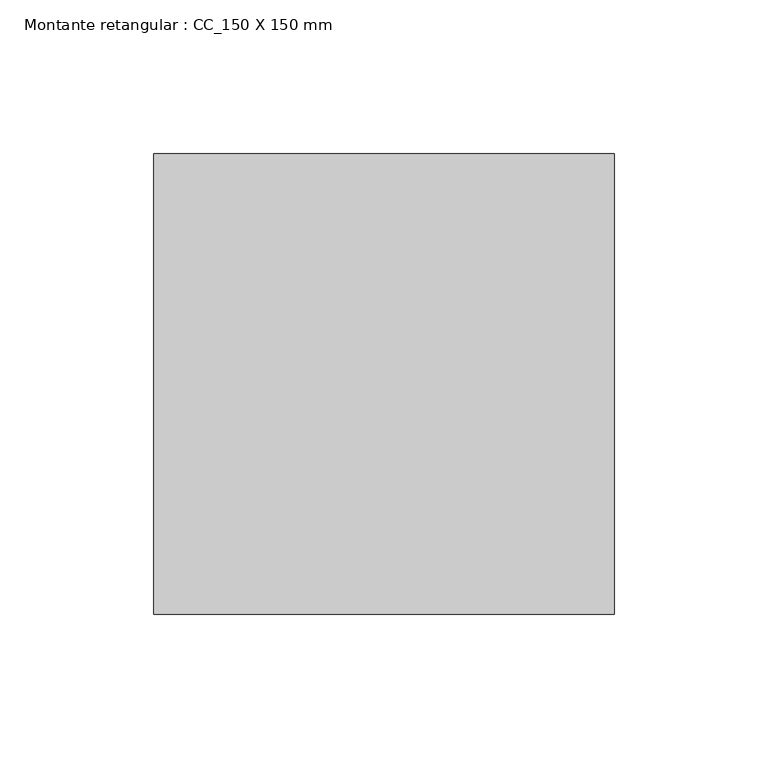
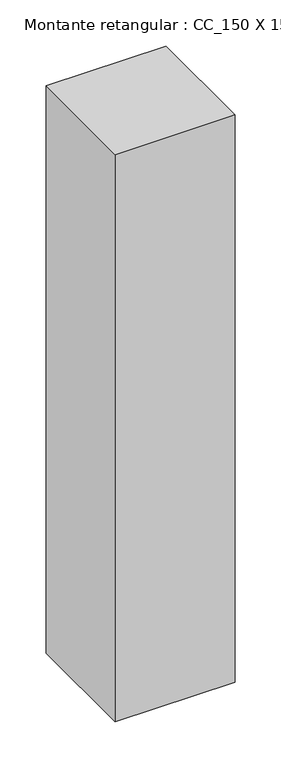
"""IFC4 building model written with IfcOpenShell, lengths in millimetres: member geometry, Montante retangular : CC_150 X 150 mm."""

import ifcopenshell
import ifcopenshell.guid

model = None  # the IFC model being written
_history = None  # IfcOwnerHistory: only IFC2X3 demands one
_inside = {}  # id of a spatial element -> (the spatial element, [elements in it])
_under = {}  # id of a project, library or spatial element -> (it, [spatial elements below it])
_declared = {}  # id of a project -> (the project, [libraries it declares])
_typed = {}  # id of a type object -> (the type object, [elements of that type])
_made_of = {}  # id of a material, layer set ... -> (it, [elements and type objects made of it])


def new_model(schema):
    """Start an empty IFC model of exactly this schema.

    Asked for "IFC4X3", IfcOpenShell would pick the latest addendum, in which some entities
    have other attributes; the version numbers below select the first issue.
    IFC2X3 requires an IfcOwnerHistory on every rooted entity: one is made here for all.
    """
    global model, _history
    if schema == "IFC4X3":
        model = ifcopenshell.file(schema_version=(4, 3, 0, 0))
    else:
        model = ifcopenshell.file(schema=schema)
    _inside.clear()
    _under.clear()
    _declared.clear()
    _typed.clear()
    _made_of.clear()
    _history = None
    if model.schema == "IFC2X3":
        org = make("IfcOrganization", Name="unknown")
        user = make(
            "IfcPersonAndOrganization",
            ThePerson=make("IfcPerson", FamilyName="unknown"),
            TheOrganization=org,
        )
        app = make(
            "IfcApplication",
            ApplicationDeveloper=org,
            Version="unknown",
            ApplicationFullName="unknown",
            ApplicationIdentifier="unknown",
        )
        _history = make(
            "IfcOwnerHistory",
            OwningUser=user,
            OwningApplication=app,
            ChangeAction="ADDED",
            CreationDate=0,
        )
    return model


def make(cls, **values):
    """One entity of the class cls with the attributes given. An attribute that is None is left unset."""
    return model.create_entity(
        cls, **{name: value for name, value in values.items() if value is not None}
    )


def rooted(cls, **values):
    """An entity with a GlobalId (a new one), such as an element, a storey or a relation."""
    return make(cls, GlobalId=ifcopenshell.guid.new(), OwnerHistory=_history, **values)


def si_unit(unit_type, name, prefix=None):
    """IfcSIUnit, for example si_unit("LENGTHUNIT", "METRE", prefix="MILLI")."""
    return make("IfcSIUnit", UnitType=unit_type, Prefix=prefix, Name=name)


def assignment(units):
    """IfcUnitAssignment: the units of a project."""
    return None if units is None else make("IfcUnitAssignment", Units=units)


def point(xyz):
    """IfcCartesianPoint."""
    return None if xyz is None else make("IfcCartesianPoint", Coordinates=xyz)


def direction(xyz):
    """IfcDirection."""
    return None if xyz is None else make("IfcDirection", DirectionRatios=xyz)


def frame(location, z_axis=None, x_axis=None):
    """IfcAxis2Placement3D, a coordinate frame: its origin and axes. An axis left out is left unset."""
    return make(
        "IfcAxis2Placement3D",
        Location=point(location),
        Axis=direction(z_axis),
        RefDirection=direction(x_axis),
    )


def origin():
    """The frame at (0, 0, 0) with its axes left unset."""
    return frame((0.0, 0.0, 0.0))


def place(relative_to, where):
    """IfcLocalPlacement: puts the frame where relative to a parent placement (None: the world)."""
    return make(
        "IfcLocalPlacement", PlacementRelTo=relative_to, RelativePlacement=where
    )


def context(
    kind, dimensions, precision=None, world=None, true_north=None, identifier=None
):
    """IfcGeometricRepresentationContext, for example the 3D "Model" context."""
    return make(
        "IfcGeometricRepresentationContext",
        ContextIdentifier=identifier,
        ContextType=kind,
        CoordinateSpaceDimension=dimensions,
        Precision=precision,
        WorldCoordinateSystem=world,
        TrueNorth=true_north,
    )


def project(units=None, contexts=None):
    """IfcProject with its units and contexts."""
    return rooted(
        "IfcProject",
        Name="project",
        RepresentationContexts=contexts,
        UnitsInContext=assignment(units),
    )


def spatial(cls, under=None, at=None, **own):
    """A site, building, storey or space (cls), placed at a placement, below another one or the project."""
    s = rooted(cls, ObjectPlacement=at, **own)
    if under is not None:
        _under.setdefault(under.id(), (under, []))[1].append(s)
    return s


def polyline(points):
    """IfcPolyline through the points."""
    return make("IfcPolyline", Points=[point(p) for p in points])


def outline(outer, holes=None, kind="AREA"):
    """IfcArbitraryClosedProfileDef: a profile drawn as a closed curve; with holes, ...WithVoids."""
    if holes is None:
        return make("IfcArbitraryClosedProfileDef", ProfileType=kind, OuterCurve=outer)
    return make(
        "IfcArbitraryProfileDefWithVoids",
        ProfileType=kind,
        OuterCurve=outer,
        InnerCurves=holes,
    )


def extrude(swept, where, along, depth):
    """IfcExtrudedAreaSolid: the profile swept, set in the frame where, extruded along a direction by depth."""
    return make(
        "IfcExtrudedAreaSolid",
        SweptArea=swept,
        Position=where,
        ExtrudedDirection=direction(along),
        Depth=depth,
    )


def shape(context_of_items, identifier, shape_type, items):
    """IfcShapeRepresentation: the items that make up one representation, for example the "Body"."""
    return make(
        "IfcShapeRepresentation",
        ContextOfItems=context_of_items,
        RepresentationIdentifier=identifier,
        RepresentationType=shape_type,
        Items=items,
    )


def source(mapping_origin, context_of_items, identifier, shape_type, items):
    """IfcRepresentationMap: a shape defined once, which mapped items show again and again."""
    return make(
        "IfcRepresentationMap",
        MappingOrigin=mapping_origin,
        MappedRepresentation=shape(context_of_items, identifier, shape_type, items),
    )


def transform(
    local_origin,
    x_axis=None,
    y_axis=None,
    z_axis=None,
    scale=None,
    scale2=None,
    scale3=None,
    uniform=True,
):
    """IfcCartesianTransformationOperator3D, or its non-uniform kind. x_axis, y_axis, z_axis: its Axis1, 2, 3."""
    if uniform:
        return make(
            "IfcCartesianTransformationOperator3D",
            Axis1=direction(x_axis),
            Axis2=direction(y_axis),
            LocalOrigin=point(local_origin),
            Scale=scale,
            Axis3=direction(z_axis),
        )
    return make(
        "IfcCartesianTransformationOperator3DnonUniform",
        Axis1=direction(x_axis),
        Axis2=direction(y_axis),
        LocalOrigin=point(local_origin),
        Scale=scale,
        Axis3=direction(z_axis),
        Scale2=scale2,
        Scale3=scale3,
    )


def mapped(mapping_source, mapping_target):
    """IfcMappedItem: shows the shape of a source again, moved by a transform."""
    return make(
        "IfcMappedItem", MappingSource=mapping_source, MappingTarget=mapping_target
    )


def made_of(thing, what):
    """Note that an element or type object is made of a material, layer set ...; save() writes the relation."""
    if what is not None:
        _made_of.setdefault(what.id(), (what, []))[1].append(thing)
    return thing


def element(
    cls,
    number,
    at=None,
    inside=None,
    cuts=None,
    type_object=None,
    material=None,
    context=None,
    identifier="Body",
    shape_type=None,
    held_by="IfcProductDefinitionShape",
    body=None,
    shapes=None,
    **own,
):
    """One element of the class cls, such as IfcWall. Its Tag is "e" and its number.

    at: its placement. inside: the storey or other place that contains it. cuts: it is an
    opening in that element (IfcRelVoidsElement). A single representation is given by context,
    identifier, shape_type and body (its items); several are given by shapes. held_by: the class
    of the entity that holds the representations. save() writes the other relations.
    """
    e = rooted(cls, Tag="e%d" % number, ObjectPlacement=at, **own)
    if body is not None:
        shapes = [shape(context, identifier, shape_type, body)]
    if shapes is not None:
        e.Representation = make(held_by, Representations=shapes)
    if inside is not None:
        _inside.setdefault(inside.id(), (inside, []))[1].append(e)
    if cuts is not None:
        rooted(
            "IfcRelVoidsElement", RelatingBuildingElement=cuts, RelatedOpeningElement=e
        )
    if type_object is not None:
        _typed.setdefault(type_object.id(), (type_object, []))[1].append(e)
    return made_of(e, material)


def aggregate(whole, parts):
    """IfcRelAggregates: a whole, such as a stair, and the parts it consists of."""
    return rooted("IfcRelAggregates", RelatingObject=whole, RelatedObjects=parts)


def save(model, path):
    """Write the relations noted so far, then the file.

    IfcRelAggregates (storeys below a building ...), IfcRelContainedInSpatialStructure (elements
    in a storey), IfcRelDefinesByType, IfcRelAssociatesMaterial and IfcRelDeclares: one each for
    every whole, place, type object, material and project.
    """
    for whole, parts in _under.values():
        aggregate(whole, parts)
    for where, things in _inside.values():
        rooted(
            "IfcRelContainedInSpatialStructure",
            RelatedElements=things,
            RelatingStructure=where,
        )
    for kind, things in _typed.values():
        rooted("IfcRelDefinesByType", RelatedObjects=things, RelatingType=kind)
    for what, things in _made_of.values():
        rooted("IfcRelAssociatesMaterial", RelatedObjects=things, RelatingMaterial=what)
    for by, libraries in _declared.values():
        rooted("IfcRelDeclares", RelatingContext=by, RelatedDefinitions=libraries)
    model.write(path)


def montante_retangular_cc_150_x_150_mm_9af7129c(model_context):
    return source(origin(), model_context, "Body", "SweptSolid", [
        extrude(outline(polyline([(0.0, 75.0), (0.0, -75.0), (-150.0, -75.0), (-150.0, 75.0), (0.0, 75.0)])), frame((0.0, 0.0, -750.0), z_axis=(0.0, 0.0, 1.0), x_axis=(1.0, 0.0, 0.0)), (0.0, 0.0, 1.0), 750.0),
    ])


if __name__ == "__main__":
    model = new_model("IFC4")
    model_context = context("Model", 3, world=origin())
    ifc_project = project(units=[si_unit("LENGTHUNIT", "METRE", prefix="MILLI")], contexts=[model_context])
    site = spatial("IfcSite", under=ifc_project)
    building = spatial("IfcBuilding", under=site)
    placement = place(None, origin())
    montante_retangular_cc_150_x_150_mm_shape = montante_retangular_cc_150_x_150_mm_9af7129c(model_context)
    element("IfcMember", 1, ObjectType="Montante retangular : CC_150 X 150 mm", at=placement, inside=building, context=model_context, shape_type="MappedRepresentation", body=[
        mapped(montante_retangular_cc_150_x_150_mm_shape, transform((0.0, 0.0, 0.0), x_axis=(1.0, 0.0, 0.0), y_axis=(0.0, 1.0, 0.0), z_axis=(0.0, 0.0, 1.0))),
    ])
    save(model, "model.ifc")

# Revit data of these elements
# Type "Montante retangular : CC_150 X 150 mm"
#   built-in parameter 1007304 = 0.492126 (stored number, unit not read)
#   built-in parameter 1007301 = 0.246063 (stored number, unit not read)
#   built-in parameter 1007300 = 0.246063 (stored number, unit not read)
# Element 1 (IfcMember, "Montante retangular : CC_150 X 150 mm")
#   Materials on its faces: ".ALUMÍNIO"
# Materials
#   ".ALUMÍNIO": class "CC_METAIS", colour RGB 244 244 244, transparency 0, Description = "Material alumínio", Cost = 0
